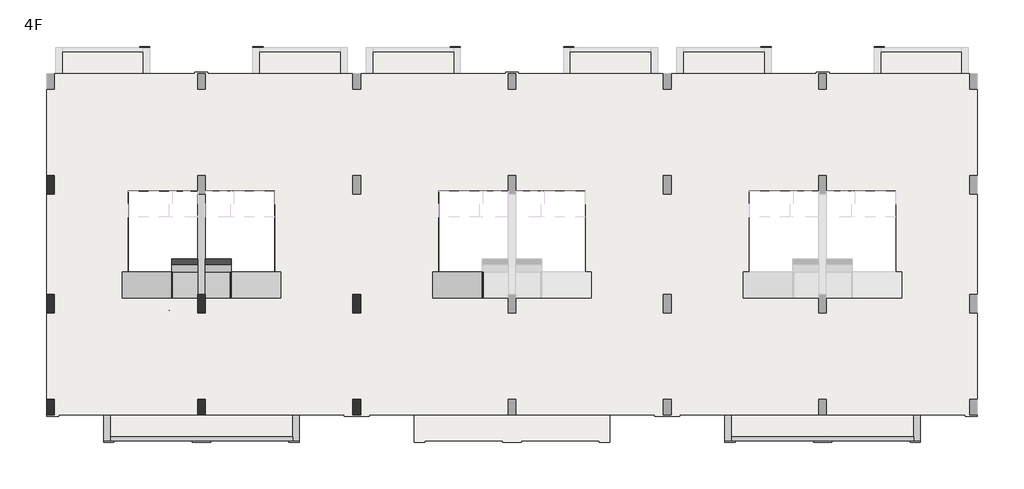
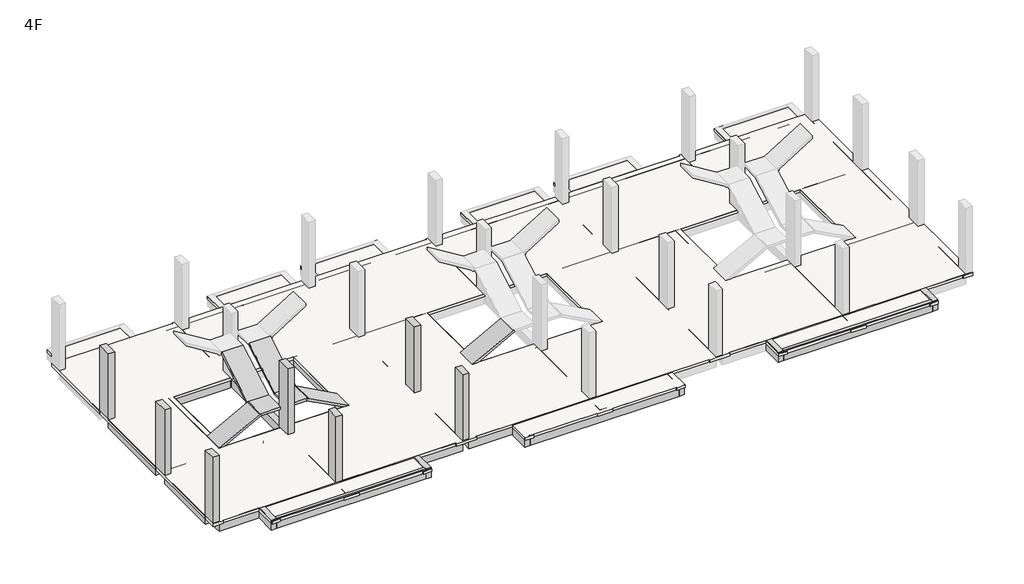
# One storey, part 1 of 3: 35 beams, 7 columns, 2 slabs.
"""IFC4 building model written with IfcOpenShell, lengths in millimetres."""

from ifc_helpers import new_model, si_unit, frame, origin, place, context, project, spatial, polyline, outline, extrude, faceted_brep, element, save

model = new_model("IFC4")

# Units and contexts
model_context = context("Model", 3, world=origin())
ifc_project = project(units=[si_unit("LENGTHUNIT", "METRE", prefix="MILLI")], contexts=[model_context])

# Site, building, storey
site = spatial("IfcSite", under=ifc_project)
building = spatial("IfcBuilding", under=site)
storey = spatial("IfcBuildingStorey", under=building, Name="4F", Elevation=10630.0)

# Beams
placement = place(None, origin())
element("IfcBeam", 1, ObjectType="M_Concrete-Rectangular Beam : 1000x120", at=placement, inside=storey, context=model_context, shape_type="Brep", body=[
    faceted_brep([(4730.4772067, 5424.9999998, 11680.0), (4730.4772067, 4424.9999998, 11680.0), (4787.1330577, 4424.9999998, 11574.2166623), (4787.1330577, 5424.9999998, 11574.2166623), (4700.0000007, 5424.9999998, 11663.6768996), (2770.0, 5424.9999998, 10630.0), (2770.0, 4424.9999998, 10630.0), (4700.0000007, 4424.9999998, 11663.6768996), (3024.1661582, 4424.9999998, 10630.0), (4760.5888269, 4424.9999998, 11560.0), (3024.1661582, 4449.9999998, 10630.0), (3020.0, 4449.9999998, 10627.7686728), (3020.0, 5424.9999998, 10627.7686728), (4760.5888269, 5424.9999998, 11560.0), (3020.0, 5424.9999998, 10630.0), (3020.0, 4449.9999998, 10630.0)], [[[0, 1, 2, 3]], [[1, 0, 4, 5, 6, 7]], [[2, 1, 7, 6, 8, 9]], [[3, 2, 9, 8, 10, 11, 12, 13]], [[0, 3, 13, 12, 14, 5, 4]], [[5, 14, 15, 10, 8, 6]], [[14, 12, 11, 15]], [[10, 15, 11]]]),
])
element("IfcBeam", 2, ObjectType="M_Concrete-Rectangular Beam : 1000x120", at=placement, inside=storey, context=model_context, shape_type="Brep", body=[
    faceted_brep([(4700.0000007, 7550.0000002, 12880.0), (5700.0000007, 7550.0000002, 12880.0), (5700.0000007, 7609.0063595, 12775.5095719), (4700.0000007, 7609.0063595, 12775.5095719), (4700.0000007, 5424.9999998, 11680.0), (4700.0000007, 5484.0063591, 11575.5095719), (5700.0000007, 5484.0063591, 11575.5095719), (5700.0000007, 5424.9999998, 11680.0), (5700.0000007, 5524.9999998, 11598.6589219), (5700.0000007, 7581.5414925, 12760.0), (4700.0000007, 5524.9999998, 11598.6589219), (4700.0000007, 7581.5414925, 12760.0)], [[[0, 1, 2, 3]], [[4, 5, 6, 7]], [[1, 0, 4, 7]], [[2, 1, 7, 6, 8, 9]], [[3, 2, 9, 8, 6, 5, 10, 11]], [[0, 3, 11, 10, 5, 4]]]),
])
element("IfcBeam", 3, ObjectType="M_Concrete-Rectangular Beam : 1000x120", at=placement, inside=storey, context=model_context, shape_type="Brep", body=[
    faceted_brep([(5700.0000007, 5524.9999998, 11560.0), (4700.0000007, 5524.9999998, 11560.0), (4700.0000007, 5524.9999998, 11598.6589219), (5700.0000007, 5524.9999998, 11598.6589219), (5700.0000007, 4424.9999998, 11560.0), (5700.0000007, 4424.9999998, 11680.0), (4730.4772067, 4424.9999998, 11680.0), (4787.1330577, 4424.9999998, 11574.2166623), (4760.5888269, 4424.9999998, 11560.0), (5700.0000007, 5424.9999998, 11680.0), (4700.0000007, 5424.9999998, 11680.0), (4700.0000007, 4424.9999998, 11680.0), (5700.0000007, 5484.0063591, 11575.5095719), (4760.5888269, 5424.9999998, 11560.0), (4700.0000007, 5424.9999998, 11560.0), (4700.0000007, 4424.9999998, 11663.6768996), (4700.0000007, 5484.0063591, 11575.5095719), (4700.0000007, 5424.9999998, 11663.6768996), (4730.4772067, 5424.9999998, 11680.0), (4787.1330577, 5424.9999998, 11574.2166623)], [[[0, 1, 2, 3]], [[4, 5, 6, 7, 8]], [[6, 5, 9, 10, 11]], [[5, 4, 0, 3, 12, 9]], [[1, 0, 4, 8, 13, 14]], [[15, 11, 10, 16, 2, 1, 14, 17]], [[6, 18, 19, 7]], [[18, 6, 15, 17]], [[7, 19, 13, 8]], [[19, 18, 17, 14, 13]], [[11, 15, 6]], [[12, 16, 10, 9]], [[16, 12, 3, 2]]]),
])
element("IfcBeam", 4, ObjectType="M_Concrete-Rectangular Beam : 1000x120", at=placement, inside=storey, context=model_context, shape_type="Brep", body=[
    faceted_brep([(6969.5227948, 4424.9999998, 11680.0), (6969.5227948, 5424.9999998, 11680.0), (6912.8669437, 5424.9999998, 11574.2166623), (6912.8669437, 4424.9999998, 11574.2166623), (7000.0000007, 4424.9999998, 11663.6768996), (8930.0000014, 4424.9999998, 10630.0), (8930.0000014, 5424.9999998, 10630.0), (7000.0000007, 5424.9999998, 11663.6768996), (6939.4111745, 4424.9999998, 11560.0), (8675.8338433, 4424.9999998, 10630.0), (6939.4111745, 5424.9999998, 11560.0), (8680.0, 5424.9999998, 10627.7686736), (8680.0, 4449.9999998, 10627.7686736), (8675.8338433, 4449.9999998, 10630.0), (8680.0, 5424.9999998, 10630.0), (8680.0, 4449.9999998, 10630.0)], [[[0, 1, 2, 3]], [[1, 0, 4, 5, 6, 7]], [[0, 3, 8, 9, 5, 4]], [[3, 2, 10, 11, 12, 13, 9, 8]], [[2, 1, 7, 6, 14, 11, 10]], [[9, 13, 15, 14, 6, 5]], [[11, 14, 15, 12]], [[15, 13, 12]]]),
])
element("IfcBeam", 5, ObjectType="M_Concrete-Rectangular Beam : 1000x120", at=placement, inside=storey, context=model_context, shape_type="Brep", body=[
    faceted_brep([(7000.0000007, 7550.0000002, 12880.0), (7000.0000007, 7609.0063595, 12775.5095719), (6000.0000007, 7609.0063595, 12775.5095719), (6000.0000007, 7550.0000002, 12880.0), (7000.0000007, 5424.9999998, 11680.0), (6000.0000007, 5424.9999998, 11680.0), (6000.0000007, 5484.0063591, 11575.5095719), (7000.0000007, 5484.0063591, 11575.5095719), (6000.0000007, 7581.5414925, 12760.0), (6000.0000007, 5524.9999998, 11598.6589219), (7000.0000007, 7581.5414925, 12760.0), (7000.0000007, 5524.9999998, 11598.6589219)], [[[0, 1, 2, 3]], [[4, 5, 6, 7]], [[3, 5, 4, 0]], [[2, 8, 9, 6, 5, 3]], [[1, 10, 11, 7, 6, 9, 8, 2]], [[0, 4, 7, 11, 10, 1]]]),
])
element("IfcBeam", 6, ObjectType="M_Concrete-Rectangular Beam : 1000x120", at=placement, inside=storey, context=model_context, shape_type="Brep", body=[
    faceted_brep([(7000.0000007, 5524.9999998, 11560.0), (6000.0000007, 5524.9999998, 11560.0), (6000.0000007, 5524.9999998, 11598.6589219), (7000.0000007, 5524.9999998, 11598.6589219), (6000.0000007, 4424.9999998, 11680.0), (6000.0000007, 4424.9999998, 11560.0), (6939.4111745, 4424.9999998, 11560.0), (6912.8669437, 4424.9999998, 11574.2166623), (6969.5227948, 4424.9999998, 11680.0), (7000.0000007, 4424.9999998, 11680.0), (7000.0000007, 5424.9999998, 11680.0), (6000.0000007, 5424.9999998, 11680.0), (6000.0000007, 5484.0063591, 11575.5095719), (7000.0000007, 5424.9999998, 11560.0), (6939.4111745, 5424.9999998, 11560.0), (7000.0000007, 4424.9999998, 11663.6768996), (7000.0000007, 5424.9999998, 11663.6768996), (7000.0000007, 5484.0063591, 11575.5095719), (6969.5227948, 5424.9999998, 11680.0), (6912.8669437, 5424.9999998, 11574.2166623)], [[[0, 1, 2, 3]], [[4, 5, 6, 7, 8]], [[8, 9, 10, 11, 4]], [[5, 4, 11, 12, 2, 1]], [[1, 0, 13, 14, 6, 5]], [[9, 15, 16, 13, 0, 3, 17, 10]], [[18, 8, 7, 19]], [[8, 18, 16, 15]], [[19, 7, 6, 14]], [[18, 19, 14, 13, 16]], [[15, 9, 8]], [[17, 12, 11, 10]], [[12, 17, 3, 2]]]),
])
element("IfcBeam", 7, ObjectType="M_Concrete-Rectangular Beam : 1000x120", at=placement, inside=storey, context=model_context, shape_type="Brep", body=[
    faceted_brep([(16730.4772117, 5424.9999998, 11680.0), (16730.4772117, 4424.9999998, 11680.0), (16787.1330628, 4424.9999998, 11574.2166623), (16787.1330628, 5424.9999998, 11574.2166623), (16700.0000058, 5424.9999998, 11663.6768996), (14770.000005, 5424.9999998, 10630.0), (14770.000005, 4424.9999998, 10630.0), (16700.0000058, 4424.9999998, 11663.6768996), (15024.1661632, 4424.9999998, 10630.0), (16760.588832, 4424.9999998, 11560.0), (15024.1661632, 4449.9999998, 10630.0), (15020.0000057, 4449.9999998, 10627.7686732), (15020.0000057, 5424.9999998, 10627.7686732), (16760.588832, 5424.9999998, 11560.0), (15020.0000057, 5424.9999998, 10630.0), (15020.0000057, 4449.9999998, 10630.0)], [[[0, 1, 2, 3]], [[1, 0, 4, 5, 6, 7]], [[2, 1, 7, 6, 8, 9]], [[3, 2, 9, 8, 10, 11, 12, 13]], [[0, 3, 13, 12, 14, 5, 4]], [[5, 14, 15, 10, 8, 6]], [[14, 12, 11, 15]], [[10, 15, 11]]]),
])
element("IfcBeam", 8, ObjectType="M_Concrete-Rectangular Beam : 150x500", at=placement, inside=storey, context=model_context, shape_type="SweptSolid", body=[
    extrude(outline(polyline([(2320.0000398, -1099.9999999), (2320.0000398, -949.9999999), (9380.0000399, -949.9999999), (9380.0000399, -1099.9999999), (2320.0000398, -1099.9999999)])), frame((0.0, 0.0, 10130.0), z_axis=(0.0, 0.0, 1.0), x_axis=(1.0, 0.0, 0.0)), (0.0, 0.0, 1.0), 500.0),
])
element("IfcBeam", 9, ObjectType="M_Concrete-Rectangular Beam : 150x500", at=placement, inside=storey, context=model_context, shape_type="SweptSolid", body=[
    extrude(outline(polyline([(26320.012858, -1100.2407813), (26320.012858, -950.2407813), (33380.0128581, -950.2407813), (33380.0128581, -1100.2407813), (26320.012858, -1100.2407813)])), frame((0.0, 0.0, 10130.0), z_axis=(0.0, 0.0, 1.0), x_axis=(1.0, 0.0, 0.0)), (0.0, 0.0, 1.0), 500.0),
])
element("IfcBeam", 10, ObjectType="M_Concrete-Rectangular Beam : 150x500", at=placement, inside=storey, context=model_context, shape_type="Brep", body=[
    faceted_brep([(14320.0998335, -950.2407813, 10580.0), (14320.0998335, -1100.2407813, 10580.0), (21380.0998336, -1100.2407813, 10580.0), (21380.0998336, -950.2407813, 10580.0), (18000.0064311, -950.2407813, 10580.0), (17700.0064311, -950.2407813, 10580.0), (14320.0998335, -1100.2407813, 10080.0), (21380.0998336, -1100.2407813, 10080.0), (14320.0998335, -950.2407813, 10080.0), (21380.0998336, -950.2407813, 10080.0)], [[[0, 1, 2, 3, 4, 5]], [[1, 6, 7, 2]], [[6, 8, 9, 7]], [[8, 0, 5, 4, 3, 9]], [[1, 0, 8, 6]], [[3, 2, 7, 9]]]),
])
element("IfcBeam", 11, ObjectType="M_Concrete-Rectangular Beam : 250x400", at=placement, inside=storey, context=model_context, shape_type="Brep", body=[
    faceted_brep([(8930.0, 8549.9999993, 10630.0), (8680.0, 8549.9999993, 10630.0), (8680.0, 5424.9999998, 10630.0), (8680.0, 4449.9999998, 10630.0), (8930.0, 4449.9999998, 10630.0), (8680.0, 8549.9999993, 10488.8582236), (8680.0, 8549.9999993, 10230.0), (8680.0, 4449.9999998, 10230.0), (8680.0, 4449.9999998, 10627.7686736), (8930.0, 8549.9999993, 10230.0), (8930.0, 4449.9999998, 10230.0)], [[[0, 1, 2, 3, 4]], [[1, 5, 6, 7, 8, 3, 2]], [[6, 9, 10, 7]], [[9, 0, 4, 10]], [[1, 0, 9, 6, 5]], [[4, 3, 8, 7, 10]]]),
])
element("IfcBeam", 12, ObjectType="M_Concrete-Rectangular Beam : 250x400", at=placement, inside=storey, context=model_context, shape_type="Brep", body=[
    faceted_brep([(15020.0000057, 8549.9999993, 10630.0), (14770.0000057, 8549.9999993, 10630.0), (14770.0000057, 4449.9999998, 10630.0), (15020.0000057, 4449.9999998, 10630.0), (15020.0000057, 5424.9999998, 10630.0), (15020.0000057, 8549.9999993, 10230.0), (15020.0000057, 8549.9999993, 10488.8582241), (15020.0000057, 4449.9999998, 10627.7686732), (15020.0000057, 4449.9999998, 10230.0), (14770.0000057, 8549.9999993, 10230.0), (14770.0000057, 4449.9999998, 10230.0)], [[[0, 1, 2, 3, 4]], [[5, 6, 0, 4, 3, 7, 8]], [[9, 5, 8, 10]], [[1, 9, 10, 2]], [[1, 0, 6, 5, 9]], [[3, 2, 10, 8, 7]]]),
])
element("IfcBeam", 13, ObjectType="M_Concrete-Rectangular Beam : 250x400", at=placement, inside=storey, context=model_context, shape_type="Brep", body=[
    faceted_brep([(3020.0, 8549.9999993, 10630.0), (2770.0, 8549.9999993, 10630.0), (2770.0, 4449.9999998, 10630.0), (3020.0, 4449.9999998, 10630.0), (3020.0, 5424.9999998, 10630.0), (3020.0, 8549.9999993, 10230.0), (3020.0, 8549.9999993, 10488.8582245), (3020.0, 4449.9999998, 10627.7686728), (3020.0, 4449.9999998, 10230.0), (2770.0, 8549.9999993, 10230.0), (2770.0, 4449.9999998, 10230.0)], [[[0, 1, 2, 3, 4]], [[5, 6, 0, 4, 3, 7, 8]], [[9, 5, 8, 10]], [[1, 9, 10, 2]], [[1, 0, 6, 5, 9]], [[3, 2, 10, 8, 7]]]),
])
element("IfcBeam", 14, ObjectType="M_Concrete-Rectangular Beam : 250x500", at=placement, inside=storey, context=model_context, shape_type="Brep", body=[
    faceted_brep([(2070.0000398, -1099.9999999, 10630.0), (2320.0000398, -1099.9999999, 10630.0), (2320.0000398, -949.9999999, 10630.0), (2320.0000398, -100.0000007, 10630.0), (2070.0000398, -100.0000007, 10630.0), (2320.0000398, -1099.9999999, 10130.0), (2320.0000398, -949.9999999, 10130.0), (2320.0000398, -100.0000007, 10130.0), (2070.0000398, -1099.9999999, 10130.0), (2070.0000398, -100.0000007, 10130.0)], [[[0, 1, 2, 3, 4]], [[1, 5, 6, 7, 3, 2]], [[5, 8, 9, 7, 6]], [[8, 0, 4, 9]], [[4, 3, 7, 9]], [[1, 0, 8, 5]]]),
])
element("IfcBeam", 15, ObjectType="M_Concrete-Rectangular Beam : 250x500", at=placement, inside=storey, context=model_context, shape_type="Brep", body=[
    faceted_brep([(9380.0000399, -1099.9999999, 10630.0), (9630.0000399, -1099.9999999, 10630.0), (9630.0000399, -100.0000007, 10630.0), (9380.0000399, -100.0000007, 10630.0), (9380.0000399, -949.9999999, 10630.0), (9380.0000399, -1099.9999999, 10130.0), (9380.0000399, -100.0000007, 10130.0), (9380.0000399, -949.9999999, 10130.0), (9630.0000399, -1099.9999999, 10130.0), (9630.0000399, -100.0000007, 10130.0)], [[[0, 1, 2, 3, 4]], [[5, 0, 4, 3, 6, 7]], [[8, 5, 7, 6, 9]], [[1, 8, 9, 2]], [[1, 0, 5, 8]], [[3, 2, 9, 6]]]),
])
element("IfcBeam", 16, ObjectType="M_Concrete-Rectangular Beam : 250x500", at=placement, inside=storey, context=model_context, shape_type="Brep", body=[
    faceted_brep([(26070.012858, -1100.2407813, 10630.0), (26320.012858, -1100.2407813, 10630.0), (26320.012858, -950.2407813, 10630.0), (26320.012858, -100.0000013, 10630.0), (26070.012858, -100.0000013, 10630.0), (26320.012858, -1100.2407813, 10130.0), (26320.012858, -950.2407813, 10130.0), (26320.012858, -100.0000013, 10130.0), (26070.012858, -1100.2407813, 10130.0), (26070.012858, -100.0000013, 10130.0)], [[[0, 1, 2, 3, 4]], [[1, 5, 6, 7, 3, 2]], [[5, 8, 9, 7, 6]], [[8, 0, 4, 9]], [[1, 0, 8, 5]], [[4, 3, 7, 9]]]),
])
element("IfcBeam", 17, ObjectType="M_Concrete-Rectangular Beam : 250x500", at=placement, inside=storey, context=model_context, shape_type="Brep", body=[
    faceted_brep([(33380.0128581, -1100.2407813, 10630.0), (33630.0128581, -1100.2407813, 10630.0), (33630.0128581, -100.0000013, 10630.0), (33380.0128581, -100.0000013, 10630.0), (33380.0128581, -950.2407813, 10630.0), (33380.0128581, -1100.2407813, 10130.0), (33380.0128581, -100.0000013, 10130.0), (33380.0128581, -950.2407813, 10130.0), (33630.0128581, -1100.2407813, 10130.0), (33630.0128581, -100.0000013, 10130.0)], [[[0, 1, 2, 3, 4]], [[5, 0, 4, 3, 6, 7]], [[8, 5, 7, 6, 9]], [[1, 8, 9, 2]], [[1, 0, 5, 8]], [[3, 2, 9, 6]]]),
])
element("IfcBeam", 18, ObjectType="M_Concrete-Rectangular Beam : 250x500", at=placement, inside=storey, context=model_context, shape_type="Brep", body=[
    faceted_brep([(14070.0998335, -100.0000007, 10080.0), (14070.0998335, -100.0000007, 10580.0), (14320.0998335, -100.0000007, 10580.0), (14320.0998335, -100.0000007, 10080.0), (14070.0998335, -1100.2407813, 10580.0), (14320.0998335, -1100.2407813, 10580.0), (14320.0998335, -950.2407813, 10580.0), (14320.0998335, -1100.2407813, 10080.0), (14320.0998335, -950.2407813, 10080.0), (14070.0998335, -1100.2407813, 10080.0)], [[[0, 1, 2, 3]], [[2, 1, 4, 5, 6]], [[3, 2, 6, 5, 7, 8]], [[0, 3, 8, 7, 9]], [[1, 0, 9, 4]], [[5, 4, 9, 7]]]),
])
element("IfcBeam", 19, ObjectType="M_Concrete-Rectangular Beam : 250x500", at=placement, inside=storey, context=model_context, shape_type="Brep", body=[
    faceted_brep([(21630.0998336, -100.0000007, 10580.0), (21630.0998336, -100.0000007, 10080.0), (21380.0998336, -100.0000007, 10080.0), (21380.0998336, -100.0000007, 10580.0), (21380.0998336, -950.2407813, 10580.0), (21380.0998336, -1100.2407813, 10580.0), (21630.0998336, -1100.2407813, 10580.0), (21380.0998336, -950.2407813, 10080.0), (21380.0998336, -1100.2407813, 10080.0), (21630.0998336, -1100.2407813, 10080.0)], [[[0, 1, 2, 3]], [[0, 3, 4, 5, 6]], [[3, 2, 7, 8, 5, 4]], [[2, 1, 9, 8, 7]], [[1, 0, 6, 9]], [[6, 5, 8, 9]]]),
])
element("IfcBeam", 20, ObjectType="M_Concrete-Rectangular Beam : 300x400", at=placement, inside=storey, context=model_context, shape_type="SweptSolid", body=[
    extrude(outline(polyline([(165.0, 4550.0000002), (-135.0, 4550.0000002), (-135.0, 8450.0000002), (165.0, 8450.0000002), (165.0, 4550.0000002)])), frame((0.0, 0.0, 10230.0), z_axis=(0.0, 0.0, 1.0), x_axis=(1.0, 0.0, 0.0)), (0.0, 0.0, 1.0), 400.0),
])
element("IfcBeam", 21, ObjectType="M_Concrete-Rectangular Beam : 300x400", at=placement, inside=storey, context=model_context, shape_type="SweptSolid", body=[
    extrude(outline(polyline([(165.0, 500.0), (-135.0, 500.0), (-135.0, 3850.0000002), (165.0, 3850.0000002), (165.0, 500.0)])), frame((0.0, 0.0, 10230.0), z_axis=(0.0, 0.0, 1.0), x_axis=(1.0, 0.0, 0.0)), (0.0, 0.0, 1.0), 400.0),
])
element("IfcBeam", 22, ObjectType="M_Concrete-Rectangular Beam : 300x400", at=placement, inside=storey, context=model_context, shape_type="SweptSolid", body=[
    extrude(outline(polyline([(12000.0000027, 4550.0000002), (11700.0000027, 4550.0000002), (11700.0000027, 8450.0000002), (12000.0000027, 8450.0000002), (12000.0000027, 4550.0000002)])), frame((0.0, 0.0, 10230.0), z_axis=(0.0, 0.0, 1.0), x_axis=(1.0, 0.0, 0.0)), (0.0, 0.0, 1.0), 400.0),
])
element("IfcBeam", 23, ObjectType="M_Concrete-Rectangular Beam : 300x400", at=placement, inside=storey, context=model_context, shape_type="SweptSolid", body=[
    extrude(outline(polyline([(6000.0, 4550.0000002), (5700.0, 4550.0000002), (5700.0, 8450.0000002), (6000.0, 8450.0000002), (6000.0, 4550.0000002)])), frame((0.0, 0.0, 10230.0), z_axis=(0.0, 0.0, 1.0), x_axis=(1.0, 0.0, 0.0)), (0.0, 0.0, 1.0), 400.0),
])
element("IfcBeam", 24, ObjectType="M_Concrete-Rectangular Beam : 300x400", at=placement, inside=storey, context=model_context, shape_type="SweptSolid", body=[
    extrude(outline(polyline([(6000.0000007, 500.0), (5700.0000007, 500.0), (5700.0000007, 3850.0000002), (6000.0000007, 3850.0000002), (6000.0000007, 500.0)])), frame((0.0, 0.0, 10230.0), z_axis=(0.0, 0.0, 1.0), x_axis=(1.0, 0.0, 0.0)), (0.0, 0.0, 1.0), 400.0),
])
element("IfcBeam", 25, ObjectType="M_Concrete-Rectangular Beam : 300x400", at=placement, inside=storey, context=model_context, shape_type="SweptSolid", body=[
    extrude(outline(polyline([(12000.0000034, 500.0), (11700.0000034, 500.0), (11700.0000034, 3850.0000002), (12000.0000034, 3850.0000002), (12000.0000034, 500.0)])), frame((0.0, 0.0, 10230.0), z_axis=(0.0, 0.0, 1.0), x_axis=(1.0, 0.0, 0.0)), (0.0, 0.0, 1.0), 400.0),
])
element("IfcBeam", 26, ObjectType="M_Concrete-Rectangular Beam : 300x400", at=placement, inside=storey, context=model_context, shape_type="Brep", body=[
    faceted_brep([(6000.0000007, -100.0, 10580.0), (5700.0000007, -100.0000007, 10580.0), (5700.0000007, -949.9999999, 10580.0), (6000.0000007, -949.9999999, 10580.0), (6000.0000007, -949.9999999, 10180.0), (6000.0000007, -100.0, 10180.0), (5700.0000007, -100.0000007, 10180.0), (5700.0000007, -949.9999999, 10180.0)], [[[0, 1, 2, 3]], [[3, 4, 5, 0]], [[6, 5, 4, 7]], [[1, 6, 7, 2]], [[0, 5, 6, 1]], [[3, 2, 7, 4]]]),
])
element("IfcBeam", 27, ObjectType="M_Concrete-Rectangular Beam : 300x400", at=placement, inside=storey, context=model_context, shape_type="Brep", body=[
    faceted_brep([(18000.0064311, -100.0, 10580.0), (17700.0064311, -100.0000007, 10580.0), (17700.0064311, -950.2407813, 10580.0), (18000.0064311, -950.2407813, 10580.0), (18000.0064311, -950.2407813, 10180.0), (18000.0064311, -100.0, 10180.0), (17700.0064311, -100.0000007, 10180.0), (17700.0064311, -950.2407813, 10180.0)], [[[0, 1, 2, 3]], [[3, 4, 5, 0]], [[6, 5, 4, 7]], [[1, 6, 7, 2]], [[0, 5, 6, 1]], [[3, 2, 7, 4]]]),
])
element("IfcBeam", 28, ObjectType="M_Concrete-Rectangular Beam : 300x400", at=placement, inside=storey, context=model_context, shape_type="Brep", body=[
    faceted_brep([(30000.0064292, -100.0, 10580.0), (29700.0064292, -100.0000013, 10580.0), (29700.0064292, -950.2407813, 10580.0), (30000.0064292, -950.2407813, 10580.0), (30000.0064292, -950.2407813, 10180.0), (30000.0064292, -100.0, 10180.0), (29700.0064292, -100.0000013, 10180.0), (29700.0064292, -950.2407813, 10180.0)], [[[0, 1, 2, 3]], [[3, 4, 5, 0]], [[6, 5, 4, 7]], [[1, 6, 7, 2]], [[0, 5, 6, 1]], [[3, 2, 7, 4]]]),
])
element("IfcBeam", 29, ObjectType="M_Concrete-Rectangular Beam : 300x500", at=placement, inside=storey, context=model_context, shape_type="Brep", body=[
    faceted_brep([(164.9649925, 8849.9999993, 10630.0), (164.9649925, 8549.9999993, 10630.0), (2770.0, 8549.9999993, 10630.0), (3020.0, 8549.9999993, 10630.0), (5699.9649933, 8549.9999993, 10630.0), (5699.9649933, 8849.9999993, 10630.0), (164.9649925, 8549.9999993, 10130.0), (5699.9649933, 8549.9999993, 10130.0), (164.9649925, 8849.9999993, 10130.0), (5699.9649933, 8849.9999993, 10130.0)], [[[0, 1, 2, 3, 4, 5]], [[1, 6, 7, 4, 3, 2]], [[6, 8, 9, 7]], [[8, 0, 5, 9]], [[1, 0, 8, 6]], [[5, 4, 7, 9]]]),
])
element("IfcBeam", 30, ObjectType="M_Concrete-Rectangular Beam : 300x500", at=placement, inside=storey, context=model_context, shape_type="Brep", body=[
    faceted_brep([(165.0, 4449.9999998, 10630.0), (165.0, 4149.9999998, 10630.0), (5700.0000007, 4149.9999998, 10630.0), (5700.0000007, 4449.9999998, 10630.0), (3024.1661582, 4449.9999998, 10630.0), (3020.0, 4449.9999998, 10630.0), (2770.0, 4449.9999998, 10630.0), (165.0, 4149.9999998, 10130.0), (5700.0000007, 4149.9999998, 10130.0), (165.0, 4449.9999998, 10130.0), (5700.0000007, 4449.9999998, 10130.0)], [[[0, 1, 2, 3, 4, 5, 6]], [[1, 7, 8, 2]], [[7, 9, 10, 8]], [[9, 0, 6, 5, 4, 3, 10]], [[1, 0, 9, 7]], [[3, 2, 8, 10]]]),
])
element("IfcBeam", 31, ObjectType="M_Concrete-Rectangular Beam : 300x500", at=placement, inside=storey, context=model_context, shape_type="Brep", body=[
    faceted_brep([(165.0, 199.9999993, 10630.0), (165.0, -100.0000007, 10630.0), (2070.0000398, -100.0000007, 10630.0), (2320.0000398, -100.0000007, 10630.0), (5700.0000007, -100.0000007, 10630.0), (5700.0000007, 199.9999993, 10630.0), (165.0, -100.0000007, 10130.0), (2070.0000398, -100.0000007, 10130.0), (2320.0000398, -100.0000007, 10130.0), (5700.0000007, -100.0000007, 10130.0), (165.0, 199.9999993, 10130.0), (5700.0000007, 199.9999993, 10130.0)], [[[0, 1, 2, 3, 4, 5]], [[1, 6, 7, 8, 9, 4, 3, 2]], [[6, 10, 11, 9, 8, 7]], [[10, 0, 5, 11]], [[1, 0, 10, 6]], [[5, 4, 9, 11]]]),
])
element("IfcBeam", 32, ObjectType="M_Concrete-Rectangular Beam : 300x500", at=placement, inside=storey, context=model_context, shape_type="Brep", body=[
    faceted_brep([(6000.0000007, 4449.9999998, 10630.0), (6000.0000007, 4149.9999998, 10630.0), (11700.0000034, 4149.9999998, 10630.0), (11700.0000034, 4449.9999998, 10630.0), (8930.0, 4449.9999998, 10630.0), (8680.0, 4449.9999998, 10630.0), (8675.8338433, 4449.9999998, 10630.0), (6000.0000007, 4149.9999998, 10130.0), (11700.0000034, 4149.9999998, 10130.0), (6000.0000007, 4449.9999998, 10130.0), (11700.0000034, 4449.9999998, 10130.0)], [[[0, 1, 2, 3, 4, 5, 6]], [[1, 7, 8, 2]], [[7, 9, 10, 8]], [[9, 0, 6, 5, 4, 3, 10]], [[1, 0, 9, 7]], [[3, 2, 8, 10]]]),
])
element("IfcBeam", 33, ObjectType="M_Concrete-Rectangular Beam : 300x500", at=placement, inside=storey, context=model_context, shape_type="Brep", body=[
    faceted_brep([(6000.0000007, 199.9999993, 10630.0), (6000.0000007, -100.0000007, 10630.0), (9380.0000399, -100.0000007, 10630.0), (9630.0000399, -100.0000007, 10630.0), (11700.0000034, -100.0000007, 10630.0), (11700.0000034, 199.9999993, 10630.0), (6000.0000007, -100.0000007, 10130.0), (9380.0000399, -100.0000007, 10130.0), (9630.0000399, -100.0000007, 10130.0), (11700.0000034, -100.0000007, 10130.0), (6000.0000007, 199.9999993, 10130.0), (11700.0000034, 199.9999993, 10130.0)], [[[0, 1, 2, 3, 4, 5]], [[1, 6, 7, 8, 9, 4, 3, 2]], [[6, 10, 11, 9, 8, 7]], [[10, 0, 5, 11]], [[1, 0, 10, 6]], [[5, 4, 9, 11]]]),
])
element("IfcBeam", 34, ObjectType="M_Concrete-Rectangular Beam : 300x500", at=placement, inside=storey, context=model_context, shape_type="Brep", body=[
    faceted_brep([(12000.0000027, 4449.9999998, 10630.0), (12000.0000034, 4149.9999998, 10630.0), (17700.0000058, 4149.9999998, 10630.0), (17700.0000058, 4449.9999998, 10630.0), (15024.1661632, 4449.9999998, 10630.0), (15020.0000057, 4449.9999998, 10630.0), (14770.0000057, 4449.9999998, 10630.0), (12000.0000034, 4149.9999998, 10130.0), (17700.0000058, 4149.9999998, 10130.0), (12000.0000034, 4449.9999998, 10130.0), (17700.0000058, 4449.9999998, 10130.0)], [[[0, 1, 2, 3, 4, 5, 6]], [[1, 7, 8, 2]], [[7, 9, 10, 8]], [[9, 0, 6, 5, 4, 3, 10]], [[7, 1, 0, 9]], [[3, 2, 8, 10]]]),
])
element("IfcBeam", 35, ObjectType="M_Concrete-Rectangular Beam : 300x500", at=placement, inside=storey, context=model_context, shape_type="SweptSolid", body=[
    extrude(outline(polyline([(12000.0000034, -100.0000007), (12000.0000034, 199.9999993), (17700.0000058, 199.9999993), (17700.0000058, -100.0000007), (12000.0000034, -100.0000007)])), frame((0.0, 0.0, 10130.0), z_axis=(0.0, 0.0, 1.0), x_axis=(1.0, 0.0, 0.0)), (0.0, 0.0, 1.0), 500.0),
])

# Columns
element("IfcColumn", 36, ObjectType="M_Concrete-Rectangular-Column : 300x600", at=placement, inside=storey, context=model_context, shape_type="SweptSolid", body=[
    extrude(outline(polyline([(165.0, 500.0), (165.0, -100.0), (-135.0, -100.0), (-135.0, 500.0), (165.0, 500.0)])), frame((0.0, 0.0, 10630.0), z_axis=(0.0, 0.0, 1.0), x_axis=(1.0, 0.0, 0.0)), (0.0, 0.0, 1.0), 3300.0),
])
element("IfcColumn", 37, ObjectType="M_Concrete-Rectangular-Column : 300x600", at=placement, inside=storey, context=model_context, shape_type="SweptSolid", body=[
    extrude(outline(polyline([(6000.0000007, 500.0), (6000.0000007, -100.0), (5700.0000007, -100.0), (5700.0000007, 500.0), (6000.0000007, 500.0)])), frame((0.0, 0.0, 10630.0), z_axis=(0.0, 0.0, 1.0), x_axis=(1.0, 0.0, 0.0)), (0.0, 0.0, 1.0), 3300.0),
])
element("IfcColumn", 38, ObjectType="M_Concrete-Rectangular-Column : 300x600", at=placement, inside=storey, context=model_context, shape_type="SweptSolid", body=[
    extrude(outline(polyline([(12000.0000034, 500.0), (12000.0000034, -100.0), (11700.0000034, -100.0), (11700.0000034, 500.0), (12000.0000034, 500.0)])), frame((0.0, 0.0, 10630.0), z_axis=(0.0, 0.0, 1.0), x_axis=(1.0, 0.0, 0.0)), (0.0, 0.0, 1.0), 3300.0),
])
element("IfcColumn", 39, ObjectType="M_Concrete-Rectangular-Column : 300x700", at=placement, inside=storey, context=model_context, shape_type="SweptSolid", body=[
    extrude(outline(polyline([(165.0, 4550.0000002), (165.0, 3850.0000002), (-135.0, 3850.0000002), (-135.0, 4550.0000002), (165.0, 4550.0000002)])), frame((0.0, 0.0, 10630.0), z_axis=(0.0, 0.0, 1.0), x_axis=(1.0, 0.0, 0.0)), (0.0, 0.0, 1.0), 3300.0),
])
element("IfcColumn", 40, ObjectType="M_Concrete-Rectangular-Column : 300x700", at=placement, inside=storey, context=model_context, shape_type="SweptSolid", body=[
    extrude(outline(polyline([(164.9649925, 9150.0000002), (164.9649925, 8450.0000002), (-135.0350075, 8450.0000002), (-135.0350075, 9150.0000002), (164.9649925, 9150.0000002)])), frame((0.0, 0.0, 10630.0), z_axis=(0.0, 0.0, 1.0), x_axis=(1.0, 0.0, 0.0)), (0.0, 0.0, 1.0), 3300.0),
])
element("IfcColumn", 41, ObjectType="M_Concrete-Rectangular-Column : 300x700", at=placement, inside=storey, context=model_context, shape_type="SweptSolid", body=[
    extrude(outline(polyline([(6000.0000007, 4550.0000002), (6000.0000007, 3850.0000002), (5700.0000007, 3850.0000002), (5700.0000007, 4550.0000002), (6000.0000007, 4550.0000002)])), frame((0.0, 0.0, 10630.0), z_axis=(0.0, 0.0, 1.0), x_axis=(1.0, 0.0, 0.0)), (0.0, 0.0, 1.0), 3300.0),
])
element("IfcColumn", 42, ObjectType="M_Concrete-Rectangular-Column : 300x700", at=placement, inside=storey, context=model_context, shape_type="SweptSolid", body=[
    extrude(outline(polyline([(12000.0000034, 4550.0000002), (12000.0000034, 3850.0000002), (11700.0000034, 3850.0000002), (11700.0000034, 4550.0000002), (12000.0000034, 4550.0000002)])), frame((0.0, 0.0, 10630.0), z_axis=(0.0, 0.0, 1.0), x_axis=(1.0, 0.0, 0.0)), (0.0, 0.0, 1.0), 3300.0),
])

# Slabs
element("IfcSlab", 43, ObjectType="130", at=placement, inside=storey, context=model_context, shape_type="SweptSolid", body=[
    extrude(outline(polyline([(5599.9999639, 13100.0000001), (5599.9999639, 13150.000002), (6100.0434252, 13150.000002), (6100.0434252, 13100.0000001), (17599.9999689, 13100.0000001), (17599.9999689, 13150.000002), (18100.0434303, 13150.000002), (18100.0434303, 13100.0000001), (29599.999967, 13100.0000001), (29599.999967, 13150.000002), (30100.0434284, 13150.000002), (30100.0434284, 13100.0000001), (35835.035019, 13100.0000001), (35835.035019, -149.9999998), (35369.8260953, -149.9999998), (35369.8260953, -100.0000013), (24330.0869831, -100.0000013), (24330.0869831, -150.2407826), (23370.2729083, -150.2407826), (23370.2729083, -100.0000007), (12329.7271033, -100.0000007), (12329.7271033, -150.0), (11370.0869772, -150.0), (11370.0869772, -100.0000007), (330.1739162, -100.0000007), (330.1739162, -149.9999998), (-135.0, -149.9999998), (-135.0, 13100.0000001), (5599.9999639, 13100.0000001)]), holes=[polyline([(8680.0, 4450.0000002), (8680.0, 8549.9999993), (3020.0, 8549.9999993), (3020.0, 4450.0000002), (8680.0, 4450.0000002)]), polyline([(20680.0000058, 8549.9999993), (15020.0000057, 8549.9999993), (15020.0000057, 4449.9992702), (20680.0000058, 4449.9992702), (20680.0000058, 8549.9999993)]), polyline([(32680.0000108, 8549.9999993), (27020.000004, 8549.9999993), (27020.000004, 4449.9999998), (32680.0000108, 4449.9999998), (32680.0000108, 8549.9999993)])]), frame((0.0, 0.0, 10500.0), z_axis=(0.0, 0.0, 1.0), x_axis=(1.0, 0.0, 0.0)), (0.0, 0.0, 1.0), 130.0),
])
element("IfcSlab", 44, ObjectType="130", at=placement, inside=storey, context=model_context, shape_type="SweptSolid", body=[
    extrude(outline(polyline([(2070.0000398, -1150.0000124), (2070.0000398, -100.0000003), (9630.0000399, -100.0000003), (9630.0000399, -1150.0000124), (9230.1739067, -1150.0000124), (9230.1739067, -1099.9999999), (6200.1739064, -1099.9999999), (6200.1739064, -1150.0000063), (5500.1739275, -1150.0000063), (5500.1739275, -1099.9999999), (2470.1739272, -1099.9999999), (2470.1739272, -1150.0000124), (2070.0000398, -1150.0000124)])), frame((0.0, 0.0, 10450.0), z_axis=(0.0, 0.0, 1.0), x_axis=(1.0, 0.0, 0.0)), (0.0, 0.0, 1.0), 130.0),
    extrude(outline(polyline([(225.0000002, 13100.0000001), (225.0000002, 14100.0000002), (3459.9999747, 14100.0000002), (3459.9999747, 14150.0000066), (3859.9999642, 14150.0000066), (3859.9999642, 13100.0000001), (225.0000002, 13100.0000001)])), frame((0.0, 0.0, 10450.0), z_axis=(0.0, 0.0, 1.0), x_axis=(1.0, 0.0, 0.0)), (0.0, 0.0, 1.0), 130.0),
    extrude(outline(polyline([(8240.0000277, 14150.0000066), (8240.0000277, 14100.0000002), (11475.0000013, 14100.0000002), (11475.0000013, 13100.0000001), (7840.0000372, 13100.0000001), (7840.0000372, 14150.0000066), (8240.0000277, 14150.0000066)])), frame((0.0, 0.0, 10450.0), z_axis=(0.0, 0.0, 1.0), x_axis=(1.0, 0.0, 0.0)), (0.0, 0.0, 1.0), 130.0),
    extrude(outline(polyline([(15459.9999791, 14150.0000066), (15859.9999697, 14150.0000066), (15859.9999697, 13100.0000001), (12225.0000056, 13100.0000001), (12225.0000056, 14100.0000002), (15459.9999791, 14100.0000002), (15459.9999791, 14150.0000066)])), frame((0.0, 0.0, 10450.0), z_axis=(0.0, 0.0, 1.0), x_axis=(1.0, 0.0, 0.0)), (0.0, 0.0, 1.0), 130.0),
    extrude(outline(polyline([(20240.000029, 14150.0000066), (20240.000029, 14100.0000002), (23475.0000025, 14100.0000002), (23475.0000025, 13100.0000001), (19840.0000384, 13100.0000001), (19840.0000384, 14150.0000066), (20240.000029, 14150.0000066)])), frame((0.0, 0.0, 10450.0), z_axis=(0.0, 0.0, 1.0), x_axis=(1.0, 0.0, 0.0)), (0.0, 0.0, 1.0), 130.0),
    extrude(outline(polyline([(27459.9999804, 14150.0000066), (27859.9999709, 14150.0000066), (27859.9999709, 13100.0000001), (24225.0000069, 13100.0000001), (24225.0000069, 14100.0000002), (27459.9999804, 14100.0000002), (27459.9999804, 14150.0000066)])), frame((0.0, 0.0, 10450.0), z_axis=(0.0, 0.0, 1.0), x_axis=(1.0, 0.0, 0.0)), (0.0, 0.0, 1.0), 130.0),
    extrude(outline(polyline([(35474.9001759, 13100.0000001), (31839.9002118, 13100.0000001), (31839.9002118, 14150.0000066), (32240.000038, 14150.0000066), (32240.000038, 14100.0000002), (35474.9001759, 14100.0000002), (35474.9001759, 13100.0000001)])), frame((0.0, 0.0, 10450.0), z_axis=(0.0, 0.0, 1.0), x_axis=(1.0, 0.0, 0.0)), (0.0, 0.0, 1.0), 130.0),
    extrude(outline(polyline([(14070.0000449, -1150.0000124), (14070.0000449, -100.0000003), (21630.0000449, -100.0000003), (21630.0000449, -1150.0000124), (21230.1739117, -1150.0000124), (21230.1739117, -1099.9999999), (18200.1739114, -1099.9999999), (18200.1739114, -1150.0000063), (17500.1739325, -1150.0000063), (17500.1739325, -1099.9999999), (14470.1739322, -1099.9999999), (14470.1739322, -1150.0000124), (14070.0000449, -1150.0000124)])), frame((0.0, 0.0, 10450.0), z_axis=(0.0, 0.0, 1.0), x_axis=(1.0, 0.0, 0.0)), (0.0, 0.0, 1.0), 130.0),
    extrude(outline(polyline([(26070.000043, -1150.0000124), (26070.000043, -100.0000003), (33630.000043, -100.0000003), (33630.000043, -1150.0000124), (33230.1739098, -1150.0000124), (33230.1739098, -1099.9999999), (30200.1739095, -1099.9999999), (30200.1739095, -1150.0000063), (29500.1739306, -1150.0000063), (29500.1739306, -1099.9999999), (26470.1739303, -1099.9999999), (26470.1739303, -1150.0000124), (26070.000043, -1150.0000124)])), frame((0.0, 0.0, 10450.0), z_axis=(0.0, 0.0, 1.0), x_axis=(1.0, 0.0, 0.0)), (0.0, 0.0, 1.0), 130.0),
])

save(model, "model.ifc")

# Revit data of these elements
# Type "M_Concrete-Rectangular Beam : 1000x120"
#   Length [instance default] = 1524 mm
#   b = 1000 mm
#   h = 120 mm
#   Structural Material [instance default] = Concrete, Cast-in-Place gray
#   Assembly Code = ""
# Type "M_Concrete-Rectangular Beam : 150x500"
#   Length [instance default] = 1524 mm
#   b = 150 mm
#   h = 500 mm
#   Structural Material [instance default] = Concrete, Cast-in-Place gray
#   Assembly Code = ""
# Type "M_Concrete-Rectangular Beam : 250x400"
#   Length [instance default] = 1524 mm
#   b = 250 mm
#   h = 400 mm
#   Structural Material [instance default] = Concrete, Cast-in-Place gray
#   Assembly Code = ""
# Type "M_Concrete-Rectangular Beam : 250x500"
#   Length [instance default] = 1524 mm
#   b = 250 mm
#   h = 500 mm
#   Structural Material [instance default] = Concrete, Cast-in-Place gray
#   Assembly Code = ""
# Type "M_Concrete-Rectangular Beam : 300x400"
#   Length [instance default] = 1524 mm
#   b = 300 mm
#   h = 400 mm
#   Structural Material [instance default] = Concrete, Cast-in-Place gray
#   Assembly Code = ""
# Type "M_Concrete-Rectangular Beam : 300x500"
#   Length [instance default] = 1524 mm
#   b = 300 mm
#   h = 500 mm
#   Structural Material [instance default] = Concrete, Cast-in-Place gray
#   Assembly Code = ""
# Type "M_Concrete-Rectangular-Column : 300x600"
#   b = 300 mm
#   h = 600 mm
#   Structural Material [instance default] = Concrete, Cast-in-Place gray
# Type "M_Concrete-Rectangular-Column : 300x700"
#   b = 300 mm
#   h = 700 mm
#   Structural Material [instance default] = Concrete, Cast-in-Place gray
# Type "130"
#   Function = 0
#   Layers, outside or top first: 130 mm "VM.TM1A-Concrete Wall-M250" (function 1)
# Elements 1, 4, 7 (IfcBeam, "M_Concrete-Rectangular Beam : 1000x120")
#   Comments = ""
#   COF_GEN__Name = "STAIR"
#   Structural Material = Concrete, Cast-in-Place gray
#   Phase Created = New Construction
#   Materials on its faces: "Concrete, Cast-in-Place gray"
# Elements 2, 3, 5, 6 (IfcBeam, "M_Concrete-Rectangular Beam : 1000x120")
#   COF_GEN__Name = "STAIR"
#   Structural Material = Concrete, Cast-in-Place gray
#   Phase Created = New Construction
#   Materials on its faces: "Concrete, Cast-in-Place gray"
# Elements 8, 9, 10 (IfcBeam, "M_Concrete-Rectangular Beam : 150x500")
#   Comments = ""
#   COF_CON__WorkItemNumber = "SH3-A-03F"
#   COF_GEN__Name = "DP4"
#   Structural Material = Concrete, Cast-in-Place gray
#   Phase Created = New Construction
#   Materials on its faces: "Concrete, Cast-in-Place gray"
# Elements 11, 12, 13 (IfcBeam, "M_Concrete-Rectangular Beam : 250x400")
#   Comments = ""
#   COF_CON__WorkItemNumber = "SH3-A-03F"
#   COF_GEN__Name = "DP1"
#   Structural Material = Concrete, Cast-in-Place gray
#   Phase Created = New Construction
#   Materials on its faces: "Concrete, Cast-in-Place gray"
# Elements 14, 15, 16, 17, 18, 19 (IfcBeam, "M_Concrete-Rectangular Beam : 250x500")
#   Comments = ""
#   COF_CON__WorkItemNumber = "SH3-A-03F"
#   COF_GEN__Name = "DP2A"
#   Structural Material = Concrete, Cast-in-Place gray
#   Phase Created = New Construction
#   Materials on its faces: "Concrete, Cast-in-Place gray"
# Elements 20, 21, 22, 25 (IfcBeam, "M_Concrete-Rectangular Beam : 300x400")
#   Comments = ""
#   COF_CON__WorkItemNumber = "SH3-A-03F"
#   COF_GEN__Name = "D3"
#   Structural Material = Concrete, Cast-in-Place gray
#   Phase Created = New Construction
#   Materials on its faces: "Concrete, Cast-in-Place gray"
# Elements 23, 24, 26, 27, 28 (IfcBeam, "M_Concrete-Rectangular Beam : 300x400")
#   Comments = ""
#   COF_CON__WorkItemNumber = "SH3-A-03F"
#   COF_GEN__Name = "D6"
#   Structural Material = Concrete, Cast-in-Place gray
#   Phase Created = New Construction
#   Materials on its faces: "Concrete, Cast-in-Place gray"
# Elements 29, 30, 32, 34 (IfcBeam, "M_Concrete-Rectangular Beam : 300x500")
#   Comments = ""
#   COF_CON__WorkItemNumber = "SH3-A-03F"
#   COF_GEN__Name = "D2"
#   Structural Material = Concrete, Cast-in-Place gray
#   Phase Created = New Construction
#   Materials on its faces: "Concrete, Cast-in-Place gray"
# Elements 31, 33, 35 (IfcBeam, "M_Concrete-Rectangular Beam : 300x500")
#   Comments = ""
#   COF_CON__WorkItemNumber = "SH3-A-03F"
#   COF_GEN__Name = "D1"
#   Structural Material = Concrete, Cast-in-Place gray
#   Phase Created = New Construction
#   Materials on its faces: "Concrete, Cast-in-Place gray"
# Elements 36, 37, 38 (IfcColumn, "M_Concrete-Rectangular-Column : 300x600")
#   Comments = ""
#   COF_CON__WorkItemNumber = "SH3-A-04F"
#   COF_GEN__Name = "C1"
#   Structural Material = Concrete, Cast-in-Place gray
#   Phase Created = New Construction
#   Materials on its faces: "Concrete, Cast-in-Place gray"
# Elements 39, 40 (IfcColumn, "M_Concrete-Rectangular-Column : 300x700")
#   Comments = ""
#   COF_CON__WorkItemNumber = "SH3-A-04F"
#   COF_GEN__Name = "C3"
#   Structural Material = Concrete, Cast-in-Place gray
#   Phase Created = New Construction
#   Materials on its faces: "Concrete, Cast-in-Place gray"
# Element 41 (IfcColumn, "M_Concrete-Rectangular-Column : 300x700")
#   Comments = ""
#   COF_CON__WorkItemNumber = "SH3-A-04F"
#   COF_GEN__Name = "C4"
#   Structural Material = Concrete, Cast-in-Place gray
#   Phase Created = New Construction
#   Materials on its faces: "Concrete, Cast-in-Place gray"
# Element 42 (IfcColumn, "M_Concrete-Rectangular-Column : 300x700")
#   Comments = ""
#   COF_CON__WorkItemNumber = "SH3-A-04F"
#   COF_GEN__Name = "C5"
#   Structural Material = Concrete, Cast-in-Place gray
#   Phase Created = New Construction
#   Materials on its faces: "Concrete, Cast-in-Place gray"
# Element 43 (IfcSlab, "130")
#   COF_CON__WorkItemNumber = "SH3-A-03F"
#   COF_GEN__Name = "T130"
#   Height Offset From Level = 0 mm
#   Phase Created = New Construction
#   Materials on its faces: "VM.TM1A-Concrete Wall-M250"
# Element 44 (IfcSlab, "130")
#   COF_CON__WorkItemNumber = "SH3-A-03F"
#   COF_GEN__Name = "T130"
#   Height Offset From Level = -50 mm
#   Phase Created = New Construction
#   Materials on its faces: "VM.TM1A-Concrete Wall-M250"
# Materials
#   "Concrete, Cast-in-Place gray": class "Concrete", colour RGB 207 208 204, transparency 0, Description = "Cast-in-place concrete", Cost = 0
#   "VM.TM1A-Concrete Wall-M250": class "Concrete", colour RGB 192 192 192, transparency 0, Description = "Cast-in-place concrete", Cost = 0
